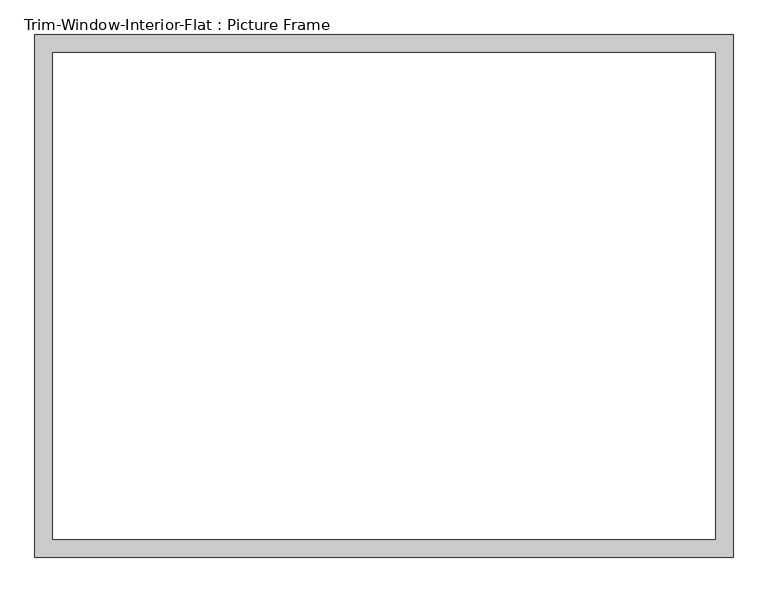
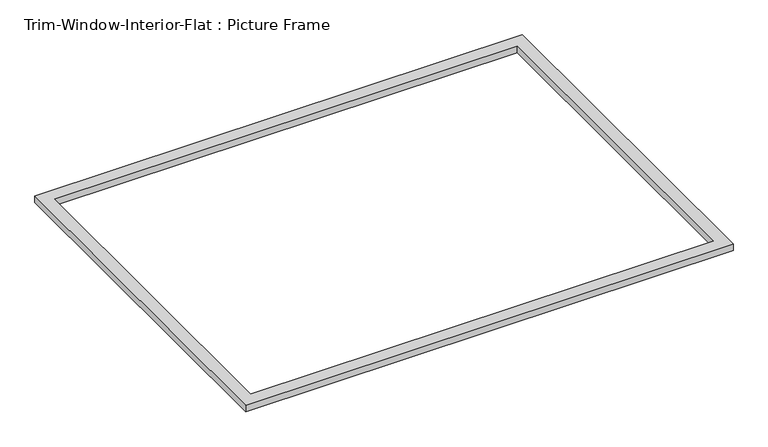
"""IFC4 building model written with IfcOpenShell, lengths in millimetres: proxy geometry, Trim-Window-Interior-Flat : Picture Frame."""

import ifcopenshell
import ifcopenshell.guid

model = None  # the IFC model being written
_history = None  # IfcOwnerHistory: only IFC2X3 demands one
_inside = {}  # id of a spatial element -> (the spatial element, [elements in it])
_under = {}  # id of a project, library or spatial element -> (it, [spatial elements below it])
_declared = {}  # id of a project -> (the project, [libraries it declares])
_typed = {}  # id of a type object -> (the type object, [elements of that type])
_made_of = {}  # id of a material, layer set ... -> (it, [elements and type objects made of it])


def new_model(schema):
    """Start an empty IFC model of exactly this schema.

    Asked for "IFC4X3", IfcOpenShell would pick the latest addendum, in which some entities
    have other attributes; the version numbers below select the first issue.
    IFC2X3 requires an IfcOwnerHistory on every rooted entity: one is made here for all.
    """
    global model, _history
    if schema == "IFC4X3":
        model = ifcopenshell.file(schema_version=(4, 3, 0, 0))
    else:
        model = ifcopenshell.file(schema=schema)
    _inside.clear()
    _under.clear()
    _declared.clear()
    _typed.clear()
    _made_of.clear()
    _history = None
    if model.schema == "IFC2X3":
        org = make("IfcOrganization", Name="unknown")
        user = make(
            "IfcPersonAndOrganization",
            ThePerson=make("IfcPerson", FamilyName="unknown"),
            TheOrganization=org,
        )
        app = make(
            "IfcApplication",
            ApplicationDeveloper=org,
            Version="unknown",
            ApplicationFullName="unknown",
            ApplicationIdentifier="unknown",
        )
        _history = make(
            "IfcOwnerHistory",
            OwningUser=user,
            OwningApplication=app,
            ChangeAction="ADDED",
            CreationDate=0,
        )
    return model


def make(cls, **values):
    """One entity of the class cls with the attributes given. An attribute that is None is left unset."""
    return model.create_entity(
        cls, **{name: value for name, value in values.items() if value is not None}
    )


def rooted(cls, **values):
    """An entity with a GlobalId (a new one), such as an element, a storey or a relation."""
    return make(cls, GlobalId=ifcopenshell.guid.new(), OwnerHistory=_history, **values)


def si_unit(unit_type, name, prefix=None):
    """IfcSIUnit, for example si_unit("LENGTHUNIT", "METRE", prefix="MILLI")."""
    return make("IfcSIUnit", UnitType=unit_type, Prefix=prefix, Name=name)


def assignment(units):
    """IfcUnitAssignment: the units of a project."""
    return None if units is None else make("IfcUnitAssignment", Units=units)


def point(xyz):
    """IfcCartesianPoint."""
    return None if xyz is None else make("IfcCartesianPoint", Coordinates=xyz)


def direction(xyz):
    """IfcDirection."""
    return None if xyz is None else make("IfcDirection", DirectionRatios=xyz)


def frame(location, z_axis=None, x_axis=None):
    """IfcAxis2Placement3D, a coordinate frame: its origin and axes. An axis left out is left unset."""
    return make(
        "IfcAxis2Placement3D",
        Location=point(location),
        Axis=direction(z_axis),
        RefDirection=direction(x_axis),
    )


def origin():
    """The frame at (0, 0, 0) with its axes left unset."""
    return frame((0.0, 0.0, 0.0))


def origin_with_axes():
    """The frame at (0, 0, 0) with the z axis (0, 0, 1) and the x axis (1, 0, 0) written out."""
    return frame((0.0, 0.0, 0.0), z_axis=(0.0, 0.0, 1.0), x_axis=(1.0, 0.0, 0.0))


def place(relative_to, where):
    """IfcLocalPlacement: puts the frame where relative to a parent placement (None: the world)."""
    return make(
        "IfcLocalPlacement", PlacementRelTo=relative_to, RelativePlacement=where
    )


def context(
    kind, dimensions, precision=None, world=None, true_north=None, identifier=None
):
    """IfcGeometricRepresentationContext, for example the 3D "Model" context."""
    return make(
        "IfcGeometricRepresentationContext",
        ContextIdentifier=identifier,
        ContextType=kind,
        CoordinateSpaceDimension=dimensions,
        Precision=precision,
        WorldCoordinateSystem=world,
        TrueNorth=true_north,
    )


def project(units=None, contexts=None):
    """IfcProject with its units and contexts."""
    return rooted(
        "IfcProject",
        Name="project",
        RepresentationContexts=contexts,
        UnitsInContext=assignment(units),
    )


def spatial(cls, under=None, at=None, **own):
    """A site, building, storey or space (cls), placed at a placement, below another one or the project."""
    s = rooted(cls, ObjectPlacement=at, **own)
    if under is not None:
        _under.setdefault(under.id(), (under, []))[1].append(s)
    return s


def polyline(points):
    """IfcPolyline through the points."""
    return make("IfcPolyline", Points=[point(p) for p in points])


def outline(outer, holes=None, kind="AREA"):
    """IfcArbitraryClosedProfileDef: a profile drawn as a closed curve; with holes, ...WithVoids."""
    if holes is None:
        return make("IfcArbitraryClosedProfileDef", ProfileType=kind, OuterCurve=outer)
    return make(
        "IfcArbitraryProfileDefWithVoids",
        ProfileType=kind,
        OuterCurve=outer,
        InnerCurves=holes,
    )


def extrude(swept, where, along, depth):
    """IfcExtrudedAreaSolid: the profile swept, set in the frame where, extruded along a direction by depth."""
    return make(
        "IfcExtrudedAreaSolid",
        SweptArea=swept,
        Position=where,
        ExtrudedDirection=direction(along),
        Depth=depth,
    )


def shape(context_of_items, identifier, shape_type, items):
    """IfcShapeRepresentation: the items that make up one representation, for example the "Body"."""
    return make(
        "IfcShapeRepresentation",
        ContextOfItems=context_of_items,
        RepresentationIdentifier=identifier,
        RepresentationType=shape_type,
        Items=items,
    )


def source(mapping_origin, context_of_items, identifier, shape_type, items):
    """IfcRepresentationMap: a shape defined once, which mapped items show again and again."""
    return make(
        "IfcRepresentationMap",
        MappingOrigin=mapping_origin,
        MappedRepresentation=shape(context_of_items, identifier, shape_type, items),
    )


def transform(
    local_origin,
    x_axis=None,
    y_axis=None,
    z_axis=None,
    scale=None,
    scale2=None,
    scale3=None,
    uniform=True,
):
    """IfcCartesianTransformationOperator3D, or its non-uniform kind. x_axis, y_axis, z_axis: its Axis1, 2, 3."""
    if uniform:
        return make(
            "IfcCartesianTransformationOperator3D",
            Axis1=direction(x_axis),
            Axis2=direction(y_axis),
            LocalOrigin=point(local_origin),
            Scale=scale,
            Axis3=direction(z_axis),
        )
    return make(
        "IfcCartesianTransformationOperator3DnonUniform",
        Axis1=direction(x_axis),
        Axis2=direction(y_axis),
        LocalOrigin=point(local_origin),
        Scale=scale,
        Axis3=direction(z_axis),
        Scale2=scale2,
        Scale3=scale3,
    )


def mapped(mapping_source, mapping_target):
    """IfcMappedItem: shows the shape of a source again, moved by a transform."""
    return make(
        "IfcMappedItem", MappingSource=mapping_source, MappingTarget=mapping_target
    )


def made_of(thing, what):
    """Note that an element or type object is made of a material, layer set ...; save() writes the relation."""
    if what is not None:
        _made_of.setdefault(what.id(), (what, []))[1].append(thing)
    return thing


def element(
    cls,
    number,
    at=None,
    inside=None,
    cuts=None,
    type_object=None,
    material=None,
    context=None,
    identifier="Body",
    shape_type=None,
    held_by="IfcProductDefinitionShape",
    body=None,
    shapes=None,
    **own,
):
    """One element of the class cls, such as IfcWall. Its Tag is "e" and its number.

    at: its placement. inside: the storey or other place that contains it. cuts: it is an
    opening in that element (IfcRelVoidsElement). A single representation is given by context,
    identifier, shape_type and body (its items); several are given by shapes. held_by: the class
    of the entity that holds the representations. save() writes the other relations.
    """
    e = rooted(cls, Tag="e%d" % number, ObjectPlacement=at, **own)
    if body is not None:
        shapes = [shape(context, identifier, shape_type, body)]
    if shapes is not None:
        e.Representation = make(held_by, Representations=shapes)
    if inside is not None:
        _inside.setdefault(inside.id(), (inside, []))[1].append(e)
    if cuts is not None:
        rooted(
            "IfcRelVoidsElement", RelatingBuildingElement=cuts, RelatedOpeningElement=e
        )
    if type_object is not None:
        _typed.setdefault(type_object.id(), (type_object, []))[1].append(e)
    return made_of(e, material)


def aggregate(whole, parts):
    """IfcRelAggregates: a whole, such as a stair, and the parts it consists of."""
    return rooted("IfcRelAggregates", RelatingObject=whole, RelatedObjects=parts)


def save(model, path):
    """Write the relations noted so far, then the file.

    IfcRelAggregates (storeys below a building ...), IfcRelContainedInSpatialStructure (elements
    in a storey), IfcRelDefinesByType, IfcRelAssociatesMaterial and IfcRelDeclares: one each for
    every whole, place, type object, material and project.
    """
    for whole, parts in _under.values():
        aggregate(whole, parts)
    for where, things in _inside.values():
        rooted(
            "IfcRelContainedInSpatialStructure",
            RelatedElements=things,
            RelatingStructure=where,
        )
    for kind, things in _typed.values():
        rooted("IfcRelDefinesByType", RelatedObjects=things, RelatingType=kind)
    for what, things in _made_of.values():
        rooted("IfcRelAssociatesMaterial", RelatedObjects=things, RelatingMaterial=what)
    for by, libraries in _declared.values():
        rooted("IfcRelDeclares", RelatingContext=by, RelatedDefinitions=libraries)
    model.write(path)


def trim_window_interior_flat_picture_frame_e25f2530(model_context):
    return source(origin(), model_context, "Body", "SweptSolid", [
        extrude(outline(polyline([(1111.25, 44.45), (1111.25, -1619.25), (-1111.25, -1619.25), (-1111.25, 44.45), (1111.25, 44.45)]), holes=[polyline([(1054.1, -12.7), (-1054.1, -12.7), (-1054.1, -1562.1), (1054.1, -1562.1), (1054.1, -12.7)])]), origin_with_axes(), (0.0, 0.0, 1.0), 31.75),
    ])


if __name__ == "__main__":
    model = new_model("IFC4")
    model_context = context("Model", 3, world=origin())
    ifc_project = project(units=[si_unit("LENGTHUNIT", "METRE", prefix="MILLI")], contexts=[model_context])
    site = spatial("IfcSite", under=ifc_project)
    building = spatial("IfcBuilding", under=site)
    placement = place(None, origin())
    trim_window_interior_flat_picture_frame_shape = trim_window_interior_flat_picture_frame_e25f2530(model_context)
    element("IfcBuildingElementProxy", 1, Name="Trim-Window-Interior-Flat : Picture Frame", ObjectType="Trim-Window-Interior-Flat : Picture Frame", at=placement, inside=building, context=model_context, shape_type="MappedRepresentation", body=[
        mapped(trim_window_interior_flat_picture_frame_shape, transform((0.0, 0.0, 0.0), x_axis=(1.0, 0.0, 0.0), y_axis=(0.0, 1.0, 0.0), z_axis=(0.0, 0.0, 1.0))),
    ])
    save(model, "model.ifc")

# Revit data of these elements
# Type "Trim-Window-Interior-Flat : Picture Frame"
#   Trim Thickness_Picture Frame = 0' - 1 1/4"
#   Trim Width = 0' - 2 1/4"
#   Trim Thickness_with Sill = 0' - 0 3/4"
#   Sill Thickness = 0' - 1 1/4"
#   Opening Width [instance default] = 2' - 0"
#   Opening Height [instance default] = 3' - 0"
#   Default Elevation = 4' - 0"
#   Sill = no
#   Picture Frame = yes
#   Trim Material [instance default] = none
# Element 1 (IfcBuildingElementProxy, "Trim-Window-Interior-Flat : Picture Frame")
#   Opening Width = 7' - 0"
#   Opening Height = 5' - 2"
#   Trim Material = Wood - Stained
#   Materials on its faces: "Wood - Stained"
# Materials
#   "Wood - Stained": class "Wood", colour RGB 224 178 126, transparency 0, Cost = 0
